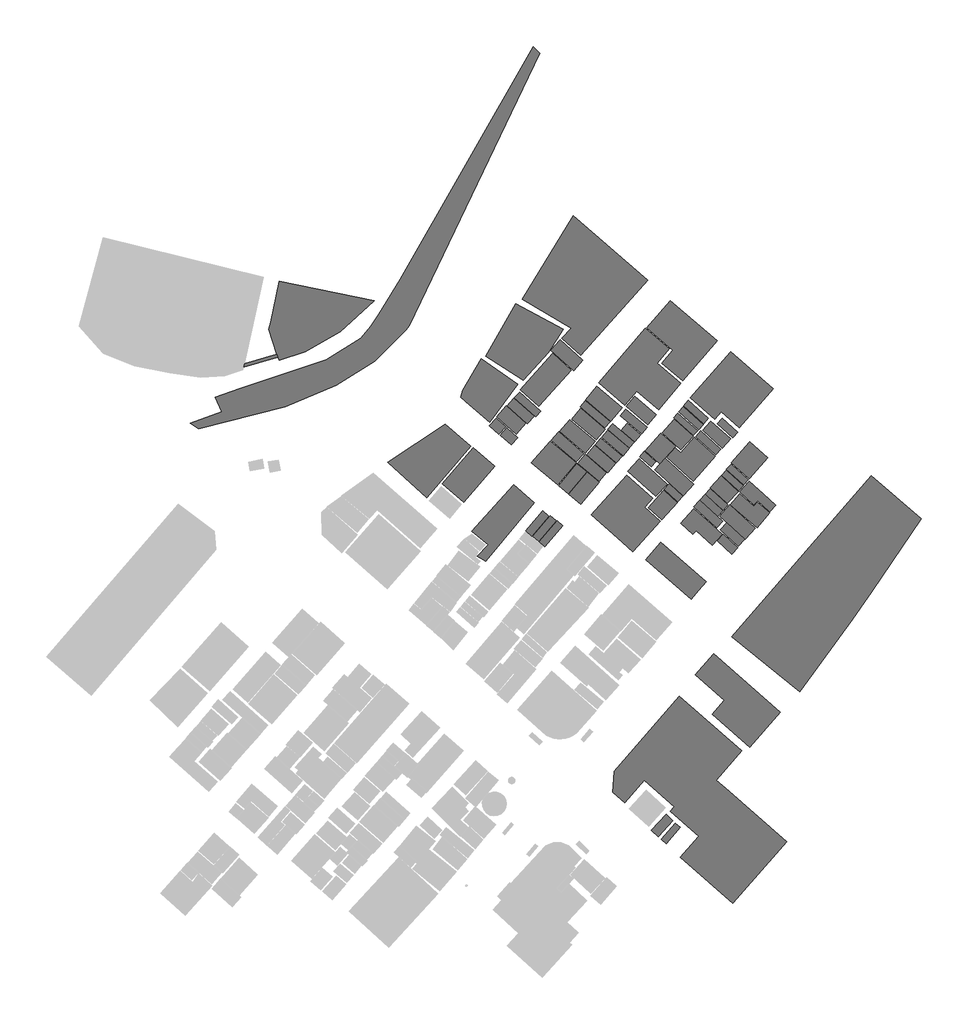
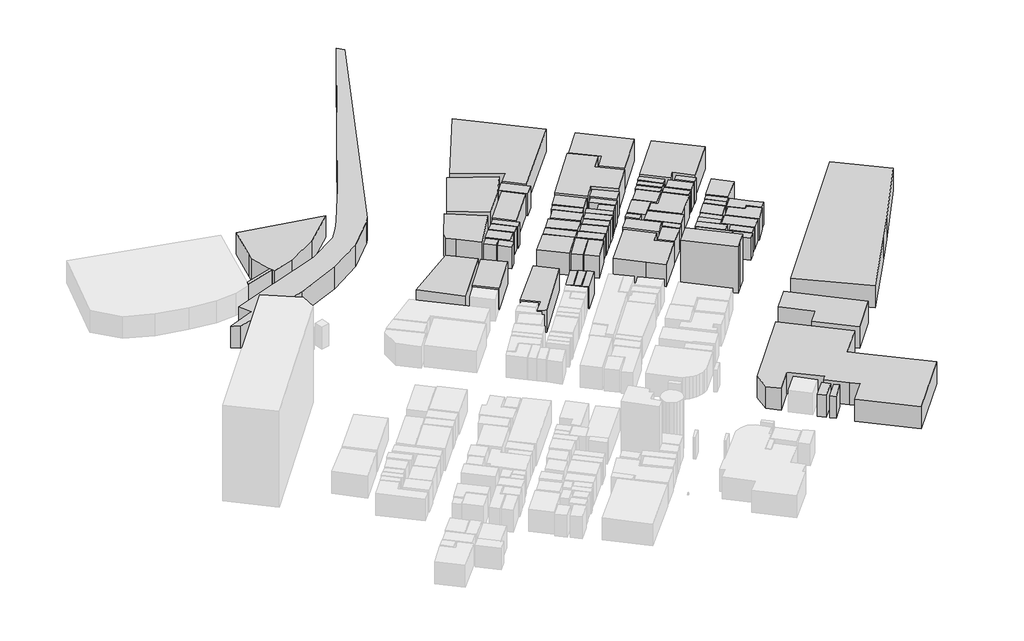
# One storey, part 3 of 3: 72 proxies.
"""IFC4 building model written with IfcOpenShell, lengths in millimetres."""

from ifc_helpers import new_model, si_unit, origin, origin_with_axes, place, context, project, spatial, polyline, outline, extrude, element, save

model = new_model("IFC4")

# Units and contexts
model_context = context("Model", 3, world=origin())
ifc_project = project(units=[si_unit("LENGTHUNIT", "METRE", prefix="MILLI")], contexts=[model_context])

# Site, building, storey
site = spatial("IfcSite", under=ifc_project)
building = spatial("IfcBuilding", under=site)
storey = spatial("IfcBuildingStorey", under=building, Name="レベル 0", Elevation=0.0)

# Proxies
placement = place(None, origin())
element("IfcBuildingElementProxy", 1, Name="Mass", at=placement, inside=storey, context=model_context, shape_type="SweptSolid", body=[
    extrude(outline(polyline([(247570.5222327, 178356.6623379), (255926.1515654, 187930.5455225), (280776.244849, 166225.2958414), (276476.4831621, 161299.3605912), (272420.6155188, 156651.4126569), (247570.5222327, 178356.6623379)])), origin_with_axes(), (0.0, 0.0, 1.0), 32000.0),
])
element("IfcBuildingElementProxy", 2, Name="Mass", at=placement, inside=storey, context=model_context, shape_type="SweptSolid", body=[
    extrude(outline(polyline([(186524.7459996, 209546.839262), (159931.2619458, 177633.895315), (155288.2419727, 180347.0515252), (161286.2288635, 186629.5648806), (152289.2485248, 193979.5495315), (175215.2887854, 219409.8292553), (186524.7459996, 209546.839262)])), origin_with_axes(), (0.0, 0.0, 1.0), 15000.0),
])
element("IfcBuildingElementProxy", 3, Name="Mass", at=placement, inside=storey, context=model_context, shape_type="SweptSolid", body=[
    extrude(outline(polyline([(258708.3503039, 38751.4319358), (262511.2907886, 35271.0307322), (254408.5886169, 26397.6755858), (250596.6150174, 29878.0767893), (258708.3503039, 38751.4319358)])), origin_with_axes(), (0.0, 0.0, 1.0), 15000.0),
])
element("IfcBuildingElementProxy", 4, Name="Mass", at=placement, inside=storey, context=model_context, shape_type="SweptSolid", body=[
    extrude(outline(polyline([(263766.8934663, 33847.7356711), (266413.5955132, 31557.1201823), (258708.3503039, 22661.5260503), (256061.6482569, 24952.1415391), (263766.8934663, 33847.7356711)])), origin_with_axes(), (0.0, 0.0, 1.0), 15000.0),
])
element("IfcBuildingElementProxy", 5, Name="Mass", at=placement, inside=storey, context=model_context, shape_type="SweptSolid", body=[
    extrude(outline(polyline([(288409.2251578, 194680.0775697), (291896.0066931, 198527.4220315), (301913.7287781, 189453.9160172), (298426.9472428, 185595.4520625), (288409.2251578, 194680.0775697)])), origin_with_axes(), (0.0, 0.0, 1.0), 15000.0),
])
element("IfcBuildingElementProxy", 6, Name="Mass", at=placement, inside=storey, context=model_context, shape_type="SweptSolid", body=[
    extrude(outline(polyline([(293955.5564102, 208390.4120248), (299230.8942796, 214483.894005), (306909.0401522, 207712.1229722), (308869.2256268, 209891.5435347), (315571.795317, 204165.0048127), (308643.3978076, 195803.1463285), (293955.5564102, 208390.4120248)])), origin_with_axes(), (0.0, 0.0, 1.0), 15000.0),
])
element("IfcBuildingElementProxy", 7, Name="Mass", at=placement, inside=storey, context=model_context, shape_type="SweptSolid", body=[
    extrude(outline(polyline([(288056.9337594, 202308.0495374), (293585.1987872, 208412.6510104), (307613.6229491, 195703.0708949), (302085.3579212, 189598.4694219), (288056.9337594, 202308.0495374)])), origin_with_axes(), (0.0, 0.0, 1.0), 15000.0),
])
element("IfcBuildingElementProxy", 8, Name="Mass", at=placement, inside=storey, context=model_context, shape_type="SweptSolid", body=[
    extrude(outline(polyline([(266016.138551, 103344.5648239), (300152.2717833, 73566.5634681), (286159.9800731, 57532.2550459), (291381.1192664, 52984.3825467), (324812.6697019, 23806.8337947), (295283.4239911, -10040.9018756), (266521.992868, 15055.7930682), (276621.0129658, 26631.1849313), (272176.7214726, 30511.8878715), (260912.4298247, 40330.3998944), (263188.7742487, 42943.4806703), (246667.2109559, 57354.3431635), (236026.2040895, 45156.2597103), (229459.1310908, 50882.798433), (230190.813227, 62280.2784138), (266016.138551, 103344.5648239)])), origin_with_axes(), (0.0, 0.0, 1.0), 15000.0),
])
element("IfcBuildingElementProxy", 9, Name="Mass", at=placement, inside=storey, context=model_context, shape_type="SweptSolid", body=[
    extrude(outline(polyline([(286801.3310816, 188664.4320382), (290098.4172494, 192300.5061393), (298155.9538572, 185006.1189515), (294858.8676895, 181370.0448504), (286801.3310816, 188664.4320382)])), origin_with_axes(), (0.0, 0.0, 1.0), 15000.0),
])
element("IfcBuildingElementProxy", 10, Name="Mass", at=placement, inside=storey, context=model_context, shape_type="SweptSolid", body=[
    extrude(outline(polyline([(371125.4389763, 224313.5255207), (398784.8303376, 200773.5595499), (371414.4985838, 160754.5054506), (360818.6572812, 145454.0835441), (332129.4910613, 105879.809151), (294768.5365618, 136180.4266618), (371125.4389763, 224313.5255207)])), origin_with_axes(), (0.0, 0.0, 1.0), 15000.0),
])
element("IfcBuildingElementProxy", 11, Name="Mass", at=placement, inside=storey, context=model_context, shape_type="SweptSolid", body=[
    extrude(outline(polyline([(45355.2593164, 291052.7204921), (45843.0474089, 289418.1550711), (26927.7092252, 283791.6917827), (27442.5966544, 285726.483506), (45355.2593164, 291052.7204921)])), origin_with_axes(), (0.0, 0.0, 1.0), 15000.0),
])
element("IfcBuildingElementProxy", 12, Name="Mass", at=placement, inside=storey, context=model_context, shape_type="SweptSolid", body=[
    extrude(outline(polyline([(321479.4510826, 94793.6749646), (304650.7619527, 75568.0721482), (284028.1654554, 93615.0087426), (290640.4040154, 101176.2637543), (274678.8937157, 115153.4660333), (284895.3442831, 126817.8138387), (321479.4510826, 94793.6749646)])), origin_with_axes(), (0.0, 0.0, 1.0), 15000.0),
])
element("IfcBuildingElementProxy", 13, Name="Mass", at=placement, inside=storey, context=model_context, shape_type="SweptSolid", body=[
    extrude(outline(polyline([(157465.2221542, 288561.9541354), (177428.401421, 274562.5128708), (162045.010339, 253624.5081838), (150672.3213364, 263331.8252796), (146237.0629554, 267490.5155365), (147212.6391378, 271371.2184759), (157465.2221542, 288561.9541354)])), origin_with_axes(), (0.0, 0.0, 1.0), 15000.0),
])
element("IfcBuildingElementProxy", 14, Name="Mass", at=placement, inside=storey, context=model_context, shape_type="SweptSolid", body=[
    extrude(outline(polyline([(41913.6433449, 308488.0849906), (46646.9944457, 331171.8500257), (98713.8565671, 320363.703156), (80105.6442205, 303306.4014085), (60720.5841739, 292442.6570756), (46728.2924611, 287872.54559), (45843.0474089, 289418.1550711), (45355.2593164, 291052.7204921), (40929.0340502, 304629.621036), (41913.6433449, 308488.0849906)])), origin_with_axes(), (0.0, 0.0, 1.0), 15000.0),
])
element("IfcBuildingElementProxy", 15, Name="Mass", at=placement, inside=storey, context=model_context, shape_type="SweptSolid", body=[
    extrude(outline(polyline([(175314.6530278, 266967.8993815), (186371.183081, 257071.5509098), (182640.5074995, 252912.8606537), (171583.9774437, 262798.0896318), (175314.6530278, 266967.8993815)])), origin_with_axes(), (0.0, 0.0, 1.0), 15000.0),
])
element("IfcBuildingElementProxy", 16, Name="Mass", at=placement, inside=storey, context=model_context, shape_type="SweptSolid", body=[
    extrude(outline(polyline([(236640.4557587, 260996.7318204), (248347.3699327, 251078.1443639), (245312.2440357, 247497.667726), (233605.3298618, 257427.3746753), (236640.4557587, 260996.7318204)])), origin_with_axes(), (0.0, 0.0, 1.0), 15000.0),
])
element("IfcBuildingElementProxy", 17, Name="Mass", at=placement, inside=storey, context=model_context, shape_type="SweptSolid", body=[
    extrude(outline(polyline([(199803.4218007, 248465.0635873), (213461.4883396, 236578.3259291), (209486.9187118, 231997.0949516), (195819.8190607, 243883.8326097), (199803.4218007, 248465.0635873)])), origin_with_axes(), (0.0, 0.0, 1.0), 15000.0),
])
element("IfcBuildingElementProxy", 18, Name="Mass", at=placement, inside=storey, context=model_context, shape_type="SweptSolid", body=[
    extrude(outline(polyline([(178458.176277, 270237.0302243), (190029.593762, 259873.6630616), (187184.1632327, 256693.4881595), (175603.7126354, 267045.7358294), (178458.176277, 270237.0302243)])), origin_with_axes(), (0.0, 0.0, 1.0), 15000.0),
])
element("IfcBuildingElementProxy", 19, Name="Mass", at=placement, inside=storey, context=model_context, shape_type="SweptSolid", body=[
    extrude(outline(polyline([(237408.2703439, 253190.8479696), (244743.1579304, 246975.0515702), (241464.1379872, 243116.5876156), (234129.2504033, 249332.384015), (237408.2703439, 253190.8479696)])), origin_with_axes(), (0.0, 0.0, 1.0), 15000.0),
])
element("IfcBuildingElementProxy", 20, Name="Mass", at=placement, inside=storey, context=model_context, shape_type="SweptSolid", body=[
    extrude(outline(polyline([(220805.4090383, 273361.6076632), (234608.005381, 261652.7818874), (228402.256893, 254325.036222), (214599.6605503, 266033.861997), (220805.4090383, 273361.6076632)])), origin_with_axes(), (0.0, 0.0, 1.0), 15000.0),
])
element("IfcBuildingElementProxy", 21, Name="Mass", at=placement, inside=storey, context=model_context, shape_type="SweptSolid", body=[
    extrude(outline(polyline([(214491.2631982, 265411.1704084), (228022.8661552, 253935.8539781), (225222.6011923, 250622.2451641), (211681.9651204, 262108.6810864), (214491.2631982, 265411.1704084)])), origin_with_axes(), (0.0, 0.0, 1.0), 15000.0),
])
element("IfcBuildingElementProxy", 22, Name="Mass", at=placement, inside=storey, context=model_context, shape_type="SweptSolid", body=[
    extrude(outline(polyline([(171051.0237899, 262709.133691), (181782.361784, 253101.8920288), (176507.0239146, 247208.5609165), (165775.6859206, 256815.8025787), (171051.0237899, 262709.133691)])), origin_with_axes(), (0.0, 0.0, 1.0), 15000.0),
])
element("IfcBuildingElementProxy", 23, Name="Mass", at=placement, inside=storey, context=model_context, shape_type="SweptSolid", body=[
    extrude(outline(polyline([(207029.9120325, 255370.268532), (212061.3558556, 261296.9581227), (225394.2303353, 249988.4340827), (220371.8196245, 244061.7444921), (207029.9120325, 255370.268532)])), origin_with_axes(), (0.0, 0.0, 1.0), 15000.0),
])
element("IfcBuildingElementProxy", 24, Name="Mass", at=placement, inside=storey, context=model_context, shape_type="SweptSolid", body=[
    extrude(outline(polyline([(247236.2970613, 238123.9354094), (255890.0191138, 247797.8940275), (263911.4232701, 240614.7017661), (255266.7343298, 230951.8626407), (247236.2970613, 238123.9354094)])), origin_with_axes(), (0.0, 0.0, 1.0), 15000.0),
])
element("IfcBuildingElementProxy", 25, Name="Mass", at=placement, inside=storey, context=model_context, shape_type="SweptSolid", body=[
    extrude(outline(polyline([(214355.7665041, 236055.7097741), (226008.4820045, 226159.3613024), (222033.9123767, 221478.0548905), (210381.1968788, 231374.4033622), (214355.7665041, 236055.7097741)])), origin_with_axes(), (0.0, 0.0, 1.0), 15000.0),
])
element("IfcBuildingElementProxy", 26, Name="Mass", at=placement, inside=storey, context=model_context, shape_type="SweptSolid", body=[
    extrude(outline(polyline([(288942.1788116, 259417.7638618), (285500.5628401, 255503.702444), (272122.5227965, 267268.125683), (294280.7484718, 292476.0155532), (317595.2125825, 271982.7905725), (298878.6028811, 250688.9621201), (288942.1788116, 259417.7638618)])), origin_with_axes(), (0.0, 0.0, 1.0), 15000.0),
])
element("IfcBuildingElementProxy", 27, Name="Mass", at=placement, inside=storey, context=model_context, shape_type="SweptSolid", body=[
    extrude(outline(polyline([(260912.4298247, 320497.137068), (286683.9006146, 298558.3780406), (267822.7611095, 276397.2291605), (256441.0389947, 286082.3072714), (262502.2576763, 293209.9020689), (248112.5090013, 305452.4634925), (260912.4298247, 320497.137068)])), origin_with_axes(), (0.0, 0.0, 1.0), 15000.0),
])
element("IfcBuildingElementProxy", 28, Name="Mass", at=placement, inside=storey, context=model_context, shape_type="SweptSolid", body=[
    extrude(outline(polyline([(259042.5754778, 234465.6223227), (263703.661678, 239680.6643824), (266684.5888963, 237011.9861434), (274164.0062865, 245373.8446268), (285717.357547, 235032.7164489), (278237.9401568, 226681.9774575), (273567.8208444, 221466.9353985), (259042.5754778, 234465.6223227)])), origin_with_axes(), (0.0, 0.0, 1.0), 15000.0),
])
element("IfcBuildingElementProxy", 29, Name="Mass", at=placement, inside=storey, context=model_context, shape_type="SweptSolid", body=[
    extrude(outline(polyline([(242530.0452973, 270815.2438433), (236017.1709747, 263142.7939044), (221690.6540905, 275318.6383721), (247191.1314975, 305330.1490734), (260524.0059747, 293999.3860486), (253830.4693967, 286115.665749), (266919.4498303, 275007.2925778), (254625.3833238, 260529.7131286), (242530.0452973, 270815.2438433)])), origin_with_axes(), (0.0, 0.0, 1.0), 15000.0),
])
element("IfcBuildingElementProxy", 30, Name="Mass", at=placement, inside=storey, context=model_context, shape_type="SweptSolid", body=[
    extrude(outline(polyline([(217788.3493659, 203008.5775755), (237236.6412034, 224747.1857341), (251454.7607328, 212026.4861259), (246947.2374512, 206989.3559493), (255474.4959245, 199361.3839816), (240533.7273711, 182659.9059996), (232006.4688979, 190287.8779672), (217788.3493659, 203008.5775755)])), origin_with_axes(), (0.0, 0.0, 1.0), 15000.0),
])
element("IfcBuildingElementProxy", 31, Name="Mass", at=placement, inside=storey, context=model_context, shape_type="SweptSolid", body=[
    extrude(outline(polyline([(257660.5092208, 216885.7044202), (260352.3768316, 219899.0869327), (267958.2578011, 213093.9574215), (265266.3901903, 210080.5749098), (257660.5092208, 216885.7044202)])), origin_with_axes(), (0.0, 0.0, 1.0), 15000.0),
])
element("IfcBuildingElementProxy", 32, Name="Mass", at=placement, inside=storey, context=model_context, shape_type="SweptSolid", body=[
    extrude(outline(polyline([(252394.2044637, 227560.4173779), (258157.330423, 234009.7231236), (273965.2778066, 219865.7284543), (268202.1518473, 213416.4227094), (252394.2044637, 227560.4173779)])), origin_with_axes(), (0.0, 0.0, 1.0), 15000.0),
])
element("IfcBuildingElementProxy", 33, Name="Mass", at=placement, inside=storey, context=model_context, shape_type="SweptSolid", body=[
    extrude(outline(polyline([(237814.760421, 226748.6944142), (243939.2108936, 233587.1824022), (259286.4695215, 219865.7284543), (253162.0190515, 213016.1209735), (237814.760421, 226748.6944142)])), origin_with_axes(), (0.0, 0.0, 1.0), 15000.0),
])
element("IfcBuildingElementProxy", 34, Name="Mass", at=placement, inside=storey, context=model_context, shape_type="SweptSolid", body=[
    extrude(outline(polyline([(176416.692787, 318662.4207782), (202441.0907354, 304763.054948), (194022.2296144, 291819.9654862), (180454.4942031, 276842.0088675), (159849.9639304, 289985.2491965), (176416.692787, 318662.4207782)])), origin_with_axes(), (0.0, 0.0, 1.0), 15000.0),
])
element("IfcBuildingElementProxy", 35, Name="Mass", at=placement, inside=storey, context=model_context, shape_type="SweptSolid", body=[
    extrude(outline(polyline([(277686.9202759, 248943.2017719), (288761.5165562, 239046.853301), (285979.3178178, 235933.395355), (274913.7546497, 245840.8633186), (277686.9202759, 248943.2017719)])), origin_with_axes(), (0.0, 0.0, 1.0), 15000.0),
])
element("IfcBuildingElementProxy", 36, Name="Mass", at=placement, inside=storey, context=model_context, shape_type="SweptSolid", body=[
    extrude(outline(polyline([(270975.3174735, 265733.6356955), (281896.3508352, 255959.601643), (279267.7150128, 253024.05558), (268346.6816511, 262798.0896318), (270975.3174735, 265733.6356955)])), origin_with_axes(), (0.0, 0.0, 1.0), 15000.0),
])
element("IfcBuildingElementProxy", 37, Name="Mass", at=placement, inside=storey, context=model_context, shape_type="SweptSolid", body=[
    extrude(outline(polyline([(223325.647506, 245485.0395531), (226667.8992376, 249421.3399565), (238456.1114295, 239424.9160513), (235113.8596954, 235488.6156479), (223325.647506, 245485.0395531)])), origin_with_axes(), (0.0, 0.0, 1.0), 15000.0),
])
element("IfcBuildingElementProxy", 38, Name="Mass", at=placement, inside=storey, context=model_context, shape_type="SweptSolid", body=[
    extrude(outline(polyline([(205394.918617, 214194.7871955), (215484.9056051, 226337.2731856), (222061.011716, 220877.6022867), (211961.9916156, 208735.1162975), (205394.918617, 214194.7871955)])), origin_with_axes(), (0.0, 0.0, 1.0), 15000.0),
])
element("IfcBuildingElementProxy", 39, Name="Mass", at=placement, inside=storey, context=model_context, shape_type="SweptSolid", body=[
    extrude(outline(polyline([(244210.2042766, 234910.4020297), (246721.409632, 237712.5141807), (252990.3899084, 232108.2898779), (250479.1845529, 229306.1777269), (244210.2042766, 234910.4020297)])), origin_with_axes(), (0.0, 0.0, 1.0), 15000.0),
])
element("IfcBuildingElementProxy", 40, Name="Mass", at=placement, inside=storey, context=model_context, shape_type="SweptSolid", body=[
    extrude(outline(polyline([(219865.9653075, 241315.2298042), (223045.6210082, 245062.4988325), (234644.1378325, 235221.747824), (231473.5152415, 231485.5982885), (219865.9653075, 241315.2298042)])), origin_with_axes(), (0.0, 0.0, 1.0), 15000.0),
])
element("IfcBuildingElementProxy", 41, Name="Mass", at=placement, inside=storey, context=model_context, shape_type="SweptSolid", body=[
    extrude(outline(polyline([(268175.052508, 262130.920072), (279150.2845483, 252312.4080491), (276684.2447567, 249554.7738685), (265709.0127164, 259373.2858914), (268175.052508, 262130.920072)])), origin_with_axes(), (0.0, 0.0, 1.0), 15000.0),
])
element("IfcBuildingElementProxy", 42, Name="Mass", at=placement, inside=storey, context=model_context, shape_type="SweptSolid", body=[
    extrude(outline(polyline([(200381.5410184, 248687.4534408), (205828.5080308, 255103.4007081), (219874.9984197, 243194.4240644), (214428.0314072, 236778.4767971), (200381.5410184, 248687.4534408)])), origin_with_axes(), (0.0, 0.0, 1.0), 15000.0),
])
element("IfcBuildingElementProxy", 43, Name="Mass", at=placement, inside=storey, context=model_context, shape_type="SweptSolid", body=[
    extrude(outline(polyline([(165513.7256498, 255970.7211358), (170807.1297437, 251233.8172607), (167058.3879376, 247041.7685262), (161764.9838411, 251789.7918941), (165513.7256498, 255970.7211358)])), origin_with_axes(), (0.0, 0.0, 1.0), 15000.0),
])
element("IfcBuildingElementProxy", 44, Name="Mass", at=placement, inside=storey, context=model_context, shape_type="SweptSolid", body=[
    extrude(outline(polyline([(199767.2893492, 218953.9300562), (209766.9452071, 230951.8626407), (215141.6473189, 226470.7070975), (205141.9914585, 214472.7745122), (199767.2893492, 218953.9300562)])), origin_with_axes(), (0.0, 0.0, 1.0), 15000.0),
])
element("IfcBuildingElementProxy", 45, Name="Mass", at=placement, inside=storey, context=model_context, shape_type="SweptSolid", body=[
    extrude(outline(polyline([(226685.9654646, 249855.0001708), (229368.7999632, 253012.9360873), (241346.7075227, 242860.8392845), (238663.8730242, 239691.7838752), (226685.9654646, 249855.0001708)])), origin_with_axes(), (0.0, 0.0, 1.0), 15000.0),
])
element("IfcBuildingElementProxy", 46, Name="Mass", at=placement, inside=storey, context=model_context, shape_type="SweptSolid", body=[
    extrude(outline(polyline([(241608.6677935, 267990.8927059), (253414.94621, 257983.3493087), (248708.6944459, 252434.7224691), (236902.4160295, 262442.2658671), (241608.6677935, 267990.8927059)])), origin_with_axes(), (0.0, 0.0, 1.0), 15000.0),
])
element("IfcBuildingElementProxy", 47, Name="Mass", at=placement, inside=storey, context=model_context, shape_type="SweptSolid", body=[
    extrude(outline(polyline([(265266.3901903, 258717.2358244), (276006.7612966, 249109.9941622), (273730.4168726, 246563.6303416), (262990.0457663, 256181.9914965), (265266.3901903, 258717.2358244)])), origin_with_axes(), (0.0, 0.0, 1.0), 15000.0),
])
element("IfcBuildingElementProxy", 48, Name="Mass", at=placement, inside=storey, context=model_context, shape_type="SweptSolid", body=[
    extrude(outline(polyline([(200562.2032737, 298903.0823133), (213109.1969412, 287683.5142149), (207969.3557633, 281934.7365073), (195422.3620984, 293165.4240985), (200562.2032737, 298903.0823133)])), origin_with_axes(), (0.0, 0.0, 1.0), 15000.0),
])
element("IfcBuildingElementProxy", 49, Name="Mass", at=placement, inside=storey, context=model_context, shape_type="SweptSolid", body=[
    extrude(outline(polyline([(215123.5810919, 235900.0368766), (219513.673909, 241070.6009659), (231039.9258277, 231307.6864062), (226649.8330131, 226126.0028249), (215123.5810919, 235900.0368766)])), origin_with_axes(), (0.0, 0.0, 1.0), 15000.0),
])
element("IfcBuildingElementProxy", 50, Name="Mass", at=placement, inside=storey, context=model_context, shape_type="SweptSolid", body=[
    extrude(outline(polyline([(263188.7742487, 255303.551576), (273558.7877295, 246029.8946938), (266910.416718, 238590.9541012), (256540.4032346, 247875.7304763), (263188.7742487, 255303.551576)])), origin_with_axes(), (0.0, 0.0, 1.0), 15000.0),
])
element("IfcBuildingElementProxy", 51, Name="Mass", at=placement, inside=storey, context=model_context, shape_type="SweptSolid", body=[
    extrude(outline(polyline([(289565.4635956, 255881.765195), (298065.6227295, 248276.0322121), (295364.7220065, 245262.6497004), (286864.56287, 252868.3826825), (289565.4635956, 255881.765195)])), origin_with_axes(), (0.0, 0.0, 1.0), 15000.0),
])
element("IfcBuildingElementProxy", 52, Name="Mass", at=placement, inside=storey, context=model_context, shape_type="SweptSolid", body=[
    extrude(outline(polyline([(249042.9196199, 206900.4000077), (257452.7476261, 216307.490802), (264868.933228, 209669.1536811), (256459.1052192, 200273.1823797), (249042.9196199, 206900.4000077)])), origin_with_axes(), (0.0, 0.0, 1.0), 15000.0),
])
element("IfcBuildingElementProxy", 53, Name="Mass", at=placement, inside=storey, context=model_context, shape_type="SweptSolid", body=[
    extrude(outline(polyline([(195332.0309707, 243361.2164547), (209351.4220203, 231652.3906789), (199198.2032438, 219498.7851968), (184781.355232, 231641.2711861), (195332.0309707, 243361.2164547)])), origin_with_axes(), (0.0, 0.0, 1.0), 15000.0),
])
element("IfcBuildingElementProxy", 54, Name="Mass", at=placement, inside=storey, context=model_context, shape_type="SweptSolid", body=[
    extrude(outline(polyline([(283323.582656, 254369.5141924), (294253.6491325, 244584.3606479), (289673.8609478, 239458.2745297), (278734.761359, 249243.4280742), (283323.582656, 254369.5141924)])), origin_with_axes(), (0.0, 0.0, 1.0), 15000.0),
])
element("IfcBuildingElementProxy", 55, Name="Mass", at=placement, inside=storey, context=model_context, shape_type="SweptSolid", body=[
    extrude(outline(polyline([(178674.9709839, 271682.564271), (196470.2031814, 291564.2171551), (206840.2166649, 282279.44078), (189044.9844673, 262397.7878959), (178674.9709839, 271682.564271)])), origin_with_axes(), (0.0, 0.0, 1.0), 15000.0),
])
element("IfcBuildingElementProxy", 56, Name="Mass", at=placement, inside=storey, context=model_context, shape_type="SweptSolid", body=[
    extrude(outline(polyline([(289240.2715339, 224658.2297926), (291778.5762287, 227449.2224516), (301109.7817413, 218998.4080266), (298571.4770465, 216196.2958756), (289240.2715339, 224658.2297926)])), origin_with_axes(), (0.0, 0.0, 1.0), 15000.0),
])
element("IfcBuildingElementProxy", 57, Name="Mass", at=placement, inside=storey, context=model_context, shape_type="SweptSolid", body=[
    extrude(outline(polyline([(185720.7989603, 191288.6323069), (195332.0309707, 202530.4393909), (198475.5542199, 199850.6416582), (188864.322212, 188597.7150823), (185720.7989603, 191288.6323069)])), origin_with_axes(), (0.0, 0.0, 1.0), 15000.0),
])
element("IfcBuildingElementProxy", 58, Name="Mass", at=placement, inside=storey, context=model_context, shape_type="SweptSolid", body=[
    extrude(outline(polyline([(181782.361784, 194168.5809067), (191122.6004089, 205087.9227036), (194455.8190282, 202241.3325814), (185115.5804033, 191321.9907845), (181782.361784, 194168.5809067)])), origin_with_axes(), (0.0, 0.0, 1.0), 15000.0),
])
element("IfcBuildingElementProxy", 59, Name="Mass", at=placement, inside=storey, context=model_context, shape_type="SweptSolid", body=[
    extrude(outline(polyline([(179894.4412126, 321264.3820621), (207897.0908602, 367032.2138689), (248699.6613337, 331672.227196), (211862.6273757, 290596.821293), (201546.8125684, 299903.8366529), (206641.4881824, 305407.9855221), (179894.4412126, 321264.3820621)])), origin_with_axes(), (0.0, 0.0, 1.0), 15000.0),
])
element("IfcBuildingElementProxy", 60, Name="Mass", at=placement, inside=storey, context=model_context, shape_type="SweptSolid", body=[
    extrude(outline(polyline([(308950.5236422, 210614.3105576), (306954.205716, 208412.6510104), (299113.4638126, 215518.006823), (304325.5698936, 221277.9040226), (312175.3449067, 214172.5482107), (318814.6828086, 208156.9026785), (315589.8615415, 204598.6650261), (308950.5236422, 210614.3105576)])), origin_with_axes(), (0.0, 0.0, 1.0), 15000.0),
])
element("IfcBuildingElementProxy", 61, Name="Mass", at=placement, inside=storey, context=model_context, shape_type="SweptSolid", body=[
    extrude(outline(polyline([(274010.4433705, 206311.0668967), (280631.7150452, 200306.5408581), (289520.2980317, 192256.0281689), (284127.5296954, 186307.0995935), (275247.9798237, 194357.6122826), (273405.2248135, 192322.7451249), (266774.9200265, 198327.2711636), (274010.4433705, 206311.0668967)])), origin_with_axes(), (0.0, 0.0, 1.0), 15000.0),
])
element("IfcBuildingElementProxy", 62, Name="Mass", at=placement, inside=storey, context=model_context, shape_type="SweptSolid", body=[
    extrude(outline(polyline([(273802.6817758, 207456.3746411), (277090.7348313, 211081.3292494), (289890.6556547, 199483.6984008), (286602.6025992, 195858.7437917), (273802.6817758, 207456.3746411)])), origin_with_axes(), (0.0, 0.0, 1.0), 15000.0),
])
element("IfcBuildingElementProxy", 63, Name="Mass", at=placement, inside=storey, context=model_context, shape_type="SweptSolid", body=[
    extrude(outline(polyline([(291868.9073563, 227882.8826658), (294371.0795995, 230640.5168464), (303738.4175612, 222145.2244511), (301245.2784328, 219387.5902697), (291868.9073563, 227882.8826658)])), origin_with_axes(), (0.0, 0.0, 1.0), 15000.0),
])
element("IfcBuildingElementProxy", 64, Name="Mass", at=placement, inside=storey, context=model_context, shape_type="SweptSolid", body=[
    extrude(outline(polyline([(282953.2250331, 217741.9053558), (288878.9470232, 224280.1670423), (298291.4505487, 215751.5161686), (292365.7285585, 209213.2544821), (282953.2250331, 217741.9053558)])), origin_with_axes(), (0.0, 0.0, 1.0), 15000.0),
])
element("IfcBuildingElementProxy", 65, Name="Mass", at=placement, inside=storey, context=model_context, shape_type="SweptSolid", body=[
    extrude(outline(polyline([(294461.4107272, 231596.7932157), (304741.0930829, 243060.9901524), (314578.15291, 234254.351962), (304298.4705543, 222779.0355325), (294461.4107272, 231596.7932157)])), origin_with_axes(), (0.0, 0.0, 1.0), 15000.0),
])
element("IfcBuildingElementProxy", 66, Name="Mass", at=placement, inside=storey, context=model_context, shape_type="SweptSolid", body=[
    extrude(outline(polyline([(277253.3308621, 211025.7317862), (280125.8607282, 214194.7871955), (289935.8212185, 205310.3125571), (287063.2913524, 202141.257147), (277253.3308621, 211025.7317862)])), origin_with_axes(), (0.0, 0.0, 1.0), 15000.0),
])
element("IfcBuildingElementProxy", 67, Name="Mass", at=placement, inside=storey, context=model_context, shape_type="SweptSolid", body=[
    extrude(outline(polyline([(280243.2911952, 214172.5482107), (282953.2250331, 217163.6917369), (292672.8543931, 208357.0535472), (289962.9205578, 205365.9100203), (280243.2911952, 214172.5482107)])), origin_with_axes(), (0.0, 0.0, 1.0), 15000.0),
])
element("IfcBuildingElementProxy", 68, Name="Mass", at=placement, inside=storey, context=model_context, shape_type="SweptSolid", body=[
    extrude(outline(polyline([(127520.453254, 212393.4293842), (106157.1415058, 231663.5101717), (137592.3740151, 252757.1877561), (151738.2286439, 240625.8212589), (127520.453254, 212393.4293842)])), origin_with_axes(), (0.0, 0.0, 1.0), 15000.0),
])
element("IfcBuildingElementProxy", 69, Name="Mass", at=placement, inside=storey, context=model_context, shape_type="SweptSolid", body=[
    extrude(outline(polyline([(135993.5130512, 219965.8038887), (152948.6657578, 239736.2618456), (164718.8117253, 229650.8819996), (147763.6590187, 209880.4240419), (135993.5130512, 219965.8038887)])), origin_with_axes(), (0.0, 0.0, 1.0), 15000.0),
])
element("IfcBuildingElementProxy", 70, Name="Mass", at=placement, inside=storey, context=model_context, shape_type="SweptSolid", body=[
    extrude(outline(polyline([(189135.315595, 188152.9353752), (198954.3091975, 199639.3712975), (202124.9317886, 196926.2150881), (192314.9712983, 185439.779165), (189135.315595, 188152.9353752)])), origin_with_axes(), (0.0, 0.0, 1.0), 15000.0),
])
element("IfcBuildingElementProxy", 71, Name="Mass", at=placement, inside=storey, context=model_context, shape_type="SweptSolid", body=[
    extrude(outline(polyline([(14949.8016656, 259362.1663986), (11481.0863548, 267457.1570581), (24777.828383, 272082.8660068), (72337.1672202, 288128.2939219), (91279.6047407, 299692.566293), (96816.9028809, 306342.0229058), (101107.6314581, 312991.4795194), (112959.0754384, 332217.0823366), (186009.8585704, 459779.902183), (189334.0440774, 455965.9161988), (117855.0225701, 306653.3687009), (115949.0357716, 304162.6023434), (99084.2141926, 287260.9734934), (77829.2997965, 274106.6136717), (49935.0475012, 262253.2344912), (2375.7086639, 250255.3019066), (-2113.7483932, 253146.3699992), (14949.8016656, 259362.1663986)])), origin_with_axes(), (0.0, 0.0, 1.0), 15000.0),
])
element("IfcBuildingElementProxy", 72, Name="Mass", at=placement, inside=storey, context=model_context, shape_type="SweptSolid", body=[
    extrude(outline(polyline([(171448.4807522, 250722.3205985), (177527.7656609, 245273.7691924), (173959.6861076, 241281.8713266), (167871.3680892, 246719.3032391), (171448.4807522, 250722.3205985)])), origin_with_axes(), (0.0, 0.0, 1.0), 15000.0),
])

save(model, "model.ifc")

# Revit data of these elements
# Elements 1, 2, 3, 4, 5, 6, 7, 8, 9, 10, 11, 12, 13, 14, 15, 16, 17, 18, 19, 20, 21, 22, 23, 24, 25, 26, 27, 28, 29, 30, 31, 32, 33, 34, 35, 36, 37, 38, 39, 40, 41, 42, 43, 44, 45, 46, 47, 48, 49, 50, 51, 52, 53, 54, 55, 56, 57, 58, 59, 60, 61, 62, 63, 64, 65, 66, 67, 68, 69, 70, 71, 72 (IfcBuildingElementProxy)
#   Phase Created = 新しい建設
#   Materials on its faces: "周辺建物"
# Materials
#   "周辺建物": class "一般", colour RGB 120 120 120, transparency 0, Cost = 0
